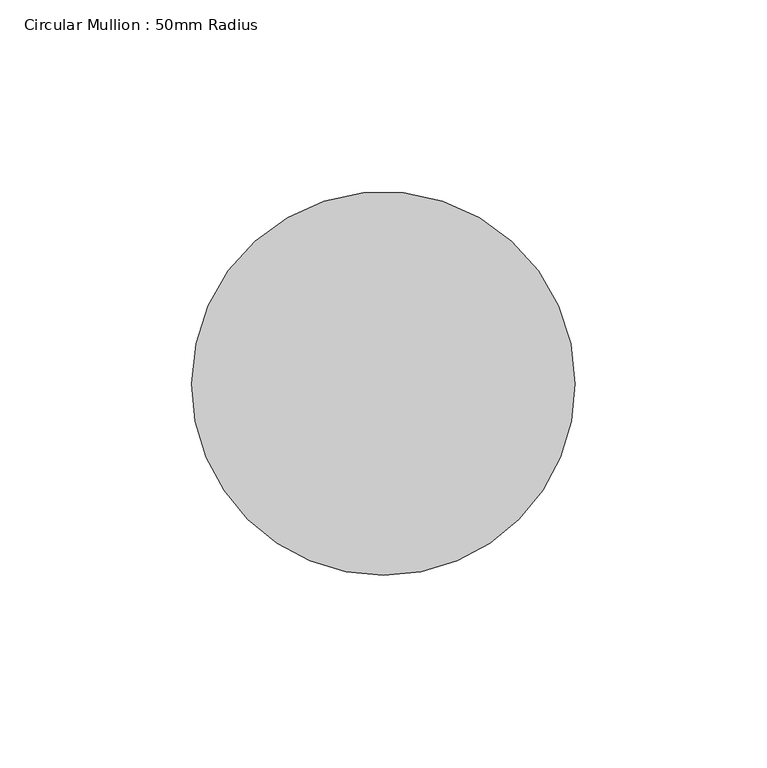
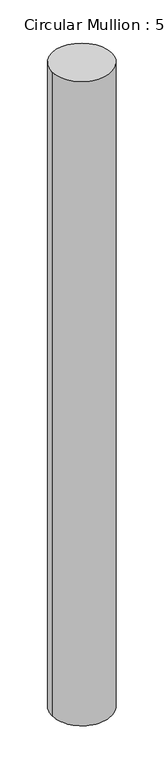
"""IFC4 building model written with IfcOpenShell, lengths in millimetres: member geometry, Circular Mullion : 50mm Radius."""

from ifc_helpers import new_model, si_unit, frame, origin, place, context, project, spatial, ellipse_curve, source, transform, mapped, element, save
from ifc_brep_helpers import plane_surface, cylinder_surface, advanced_brep


def circular_mullion_50mm_radius_53eac425(model_context):
    return source(origin(), model_context, "Body", "AdvancedBrep", [
        advanced_brep(
        [(-100.0, 0.0, 0.9040825), (0.0, 0.0, 0.0), (0.0, 0.0, -1137.5457817), (-100.0, 0.0, -1138.4144587)],
        [
            (0, 1, ellipse_curve(frame((-50.0, 0.0, 0.4520413), z_axis=(-0.009039547155433736, -0.0141757070900791, -0.9998586579690756), x_axis=(-0.5375885018471105, -0.8430397016733554, 0.01681261681830718)), 50.0070681, 50.0)),
            (1, 2),
            (2, 3, ellipse_curve(frame((-50.0, 0.0, -1137.9801202), z_axis=(-0.008685636556413167, -0.013620708825063306, 0.9998695094904699), x_axis=(0.5375943363249096, 0.8430488512299232, 0.01615437994126833)), 50.0065254, 50.0)),
            (3, 0),
            (1, 0, ellipse_curve(frame((-50.0, 0.0, 0.4520413), z_axis=(-0.009039547155433736, -0.0141757070900791, -0.9998586579690756), x_axis=(-0.5375885018471105, -0.8430397016733554, 0.01681261681830718)), 50.0070681, 50.0)),
            (3, 2, ellipse_curve(frame((-50.0, 0.0, -1137.9801202), z_axis=(-0.008685636556413167, -0.013620708825063306, 0.9998695094904699), x_axis=(0.5375943363249096, 0.8430488512299232, 0.01615437994126833)), 50.0065254, 50.0)),
        ],
        [
            cylinder_surface(frame((-50.0, 0.0, 0.0), z_axis=(0.0, 0.0, 1.0), x_axis=(1.0, 0.0, 0.0)), 50.0),
            plane_surface(frame((-256.9948252, 163.8801385, 0.0), z_axis=(0.009039547155433737, 0.014175707090079103, 0.9998586579690758), x_axis=(0.5375885018471123, 0.8430397016733544, -0.01681261681830134))),
            plane_surface(frame((-256.9948252, 163.8801385, -1137.5457817), z_axis=(0.008685636556413169, 0.01362070882506331, -0.9998695094904702), x_axis=(0.5375943363249095, 0.8430488512299231, 0.016154379941280887))),
        ],
        [
            (0, [[1, 2, 3, 4]]),
            (0, [[5, -4, 6, -2]]),
            (1, [[-1, -5]]),
            (2, [[-6, -3]]),
        ],
    ),
    ])


if __name__ == "__main__":
    model = new_model("IFC4")
    model_context = context("Model", 3, world=origin())
    ifc_project = project(units=[si_unit("LENGTHUNIT", "METRE", prefix="MILLI")], contexts=[model_context])
    site = spatial("IfcSite", under=ifc_project)
    building = spatial("IfcBuilding", under=site)
    placement = place(None, origin())
    circular_mullion_50mm_radius_shape = circular_mullion_50mm_radius_53eac425(model_context)
    element("IfcMember", 1, ObjectType="Circular Mullion : 50mm Radius", at=placement, inside=building, context=model_context, shape_type="MappedRepresentation", body=[
        mapped(circular_mullion_50mm_radius_shape, transform((0.0, 0.0, 0.0), x_axis=(1.0, 0.0, 0.0), y_axis=(0.0, 1.0, 0.0), z_axis=(0.0, 0.0, 1.0))),
    ])
    save(model, "model.ifc")

# Revit data of these elements
# Type "Circular Mullion : 50mm Radius"
#   built-in parameter 1007350 = 0.164042 (stored number, unit not read)
# Element 1 (IfcMember, "Circular Mullion : 50mm Radius")
#   Materials on its faces: "Aluminium"
# Materials
#   "Aluminium": class "Metal", colour RGB 247 247 247, transparency 0, Description = "Aluminium 6061", Cost = 0
